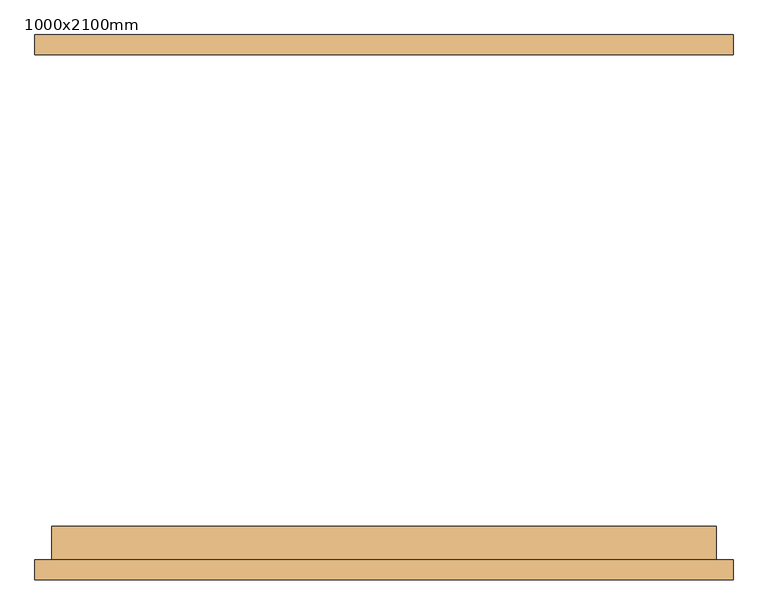
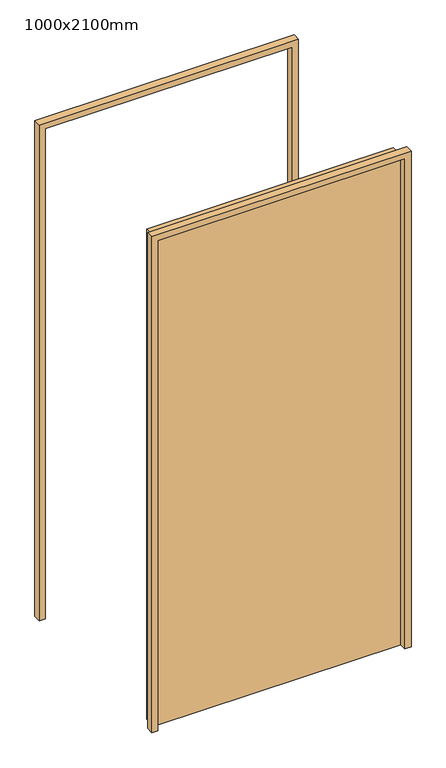
"""IFC4 building model written with IfcOpenShell, lengths in millimetres: door geometry, WWm-SingleSolid-Flush : 1000x2100mm."""

from ifc_helpers import new_model, si_unit, frame, origin, origin_with_axes, place, context, project, spatial, polyline, outline, extrude, source, transform, mapped, element, save


def door_1000x2100mm_d167f1af(model_context):
    return source(origin(), model_context, "Body", "SweptSolid", [
        extrude(outline(polyline([(2125.0, -525.0), (0.0, -525.0), (0.0, -500.0), (2100.0, -500.0), (2100.0, 500.0), (0.0, 500.0), (0.0, 525.0), (2125.0, 525.0), (2125.0, -525.0)])), frame((0.0, -410.0, 0.0), z_axis=(0.0, 1.0, 0.0), x_axis=(0.0, 0.0, 1.0)), (0.0, 0.0, 1.0), 30.0),
        extrude(outline(polyline([(2125.0, 525.0), (2125.0, -525.0), (0.0, -525.0), (0.0, -500.0), (2100.0, -500.0), (2100.0, 500.0), (0.0, 500.0), (0.0, 525.0), (2125.0, 525.0)])), frame((0.0, 380.0, 0.0), z_axis=(0.0, 1.0, 0.0), x_axis=(0.0, 0.0, 1.0)), (0.0, 0.0, 1.0), 30.0),
        extrude(outline(polyline([(500.0, -330.0), (500.0, -380.0), (-500.0, -380.0), (-500.0, -330.0), (500.0, -330.0)])), origin_with_axes(), (0.0, 0.0, 1.0), 2100.0),
    ])


if __name__ == "__main__":
    model = new_model("IFC4")
    model_context = context("Model", 3, world=origin())
    ifc_project = project(units=[si_unit("LENGTHUNIT", "METRE", prefix="MILLI")], contexts=[model_context])
    site = spatial("IfcSite", under=ifc_project)
    building = spatial("IfcBuilding", under=site)
    placement = place(None, origin())
    door_1000x2100mm_shape = door_1000x2100mm_d167f1af(model_context)
    element("IfcDoor", 1, ObjectType="WWm-SingleSolid-Flush : 1000x2100mm", at=placement, inside=building, context=model_context, shape_type="MappedRepresentation", body=[
        mapped(door_1000x2100mm_shape, transform((0.0, 0.0, 0.0), x_axis=(1.0, 0.0, 0.0), y_axis=(0.0, 1.0, 0.0), z_axis=(0.0, 0.0, 1.0))),
    ])
    save(model, "model.ifc")

# Revit data of these elements
# Type "WWm-SingleSolid-Flush : 1000x2100mm"
#   Type Mark = "EX1-51"
#   Construction Type Id = "MDOOR"
#   Assembly Code = "C1020"
#   Analytic Construction = "Metal"
#   Thickness = 50 mm
#   Thermal Resistance (R) = 0.270117 (m²·K)/W
#   Heat Transfer Coefficient (U) = 3.7021 W/(m²·K)
#   Height = 2100 mm
#   Trim Projection Ext = 30 mm
#   Trim Projection Int = 30 mm
#   Trim Width = 25 mm
#   Width = 1000 mm
#   Not 90 Degree [instance default] = no
#   90 Degree [instance default] = yes
#   Door Material = WW-EC-RGB-White
#   Frame Material = WW-EC-RGB-White
#   Visual Light Transmittance = 0
#   Solar Heat Gain Coefficient = 0
#   Function = (empty or 0)
#   Wall Closure = (empty or 0)
# Element 1 (IfcDoor, "WWm-SingleSolid-Flush : 1000x2100mm")
#   Materials on its faces: "WW-EC-RGB-White"
# Materials
#   "WW-EC-RGB-White": class "Generic", colour RGB 255 255 255, transparency 0, Comments = "If region requests off-white, swith asset color to RGB 231-228-220", Description = "Generic Color", Cost = 0
